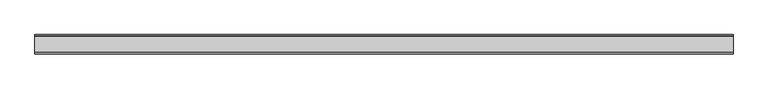
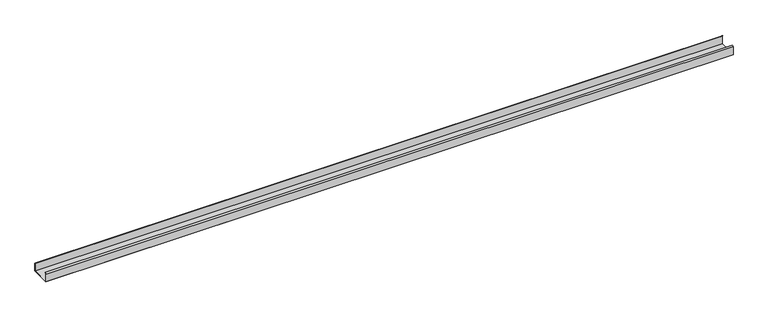
"""IFC4 building model written with IfcOpenShell, lengths in millimetres: proxy geometry, Generic Models 7:Generic Models 1:1:Generic Models 1:1 : Generic Models 7:Generic Models 1:337419:7 : Generic Models 7:Generic Models 1:1:Generic Models 1:1 : Generic Models 7:Generic Models 1:337419:306201."""

from ifc_helpers import new_model, si_unit, frame, origin, place, context, project, spatial, polyline, outline, extrude, source, transform, mapped, element, save


def generic_models_a9da2a32(model_context):
    return source(origin(), model_context, "Body", "SweptSolid", [
        extrude(outline(polyline([(-578797.4913841, 2446.5359375), (-579000.6913841, 2446.5359375), (-579000.6913841, 2535.4359375), (-578986.0982375, 2547.6810414), (-578984.3124931, 2545.5528742), (-578997.9132591, 2534.1404765), (-578997.9132591, 2449.3140625), (-578800.2695091, 2449.3140625), (-578800.2695091, 2534.1404765), (-578813.8702751, 2545.5528742), (-578812.0845307, 2547.6810414), (-578797.4913841, 2535.4359375), (-578797.4913841, 2446.5359375)])), frame((565582.1867239, 0.0, 0.0), z_axis=(1.0, 0.0, 0.0), x_axis=(0.0, 1.0, 0.0)), (0.0, 0.0, 1.0), 7315.2),
    ])


if __name__ == "__main__":
    model = new_model("IFC4")
    model_context = context("Model", 3, world=origin())
    ifc_project = project(units=[si_unit("LENGTHUNIT", "METRE", prefix="MILLI")], contexts=[model_context])
    site = spatial("IfcSite", under=ifc_project)
    building = spatial("IfcBuilding", under=site)
    placement = place(None, origin())
    generic_models_shape = generic_models_a9da2a32(model_context)
    element("IfcBuildingElementProxy", 1, Name="Generic Models 7:Generic Models 1:1:Generic Models 1:1 : Generic Models 7:Generic Models 1:337419:7 : Generic Models 7:Generic Models 1:1:Generic Models 1:1 : Generic Models 7:Generic Models 1:337419:306201", ObjectType="Generic Models 7:Generic Models 1:1:Generic Models 1:1 : Generic Models 7:Generic Models 1:337419:7 : Generic Models 7:Generic Models 1:1:Generic Models 1:1 : Generic Models 7:Generic Models 1:337419:306201", at=placement, inside=building, context=model_context, shape_type="MappedRepresentation", body=[
        mapped(generic_models_shape, transform((0.0, 0.0, 0.0), x_axis=(1.0, 0.0, 0.0), y_axis=(0.0, 1.0, 0.0), z_axis=(0.0, 0.0, 1.0))),
    ])
    save(model, "model.ifc")

# Revit data of these elements
# Type "Generic Models 7:Generic Models 1:1:Generic Models 1:1 : Generic Models 7:Generic Models 1:337419:7 : Generic Models 7:Generic Models 1:1:Generic Models 1:1 : Generic Models 7:Generic Models 1:337419:306201"
#   NameOverride = "Generic Models 7:Generic Models 1:1:Generic Models 1:1 : Generic Models 7:Generic Models 1:337419:306201"
#   ObjectTypeOverride = "Generic Models 1:1 : Generic Models 7:Generic Models 1:337419"
#   Reference = "Generic Models 1"
#   Tag = "306201"
# Element 1 (IfcBuildingElementProxy, "Generic Models 7:Generic Models 1:1:Generic Models 1:1 : Generic Models 7:Generic Models 1:337419:7 : Generic Models 7:Generic Models 1:1:Generic Models 1:1 : Generic Models 7:Generic Models 1:337419:306201")
#   Materials on its faces: "CEE' SECTION (8.0x3.5C - SEE STRUCT. DWGS)"
# Materials
#   "CEE' SECTION (8.0x3.5C - SEE STRUCT. DWGS)": class "Unassigned", colour RGB 210 209 208, transparency 0, Keynote = "M05121300.02", Cost = 0
